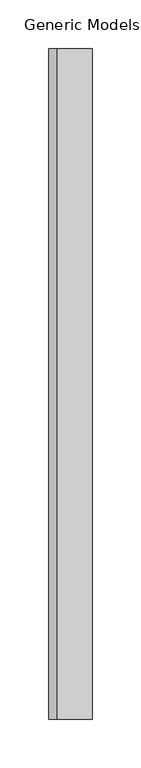
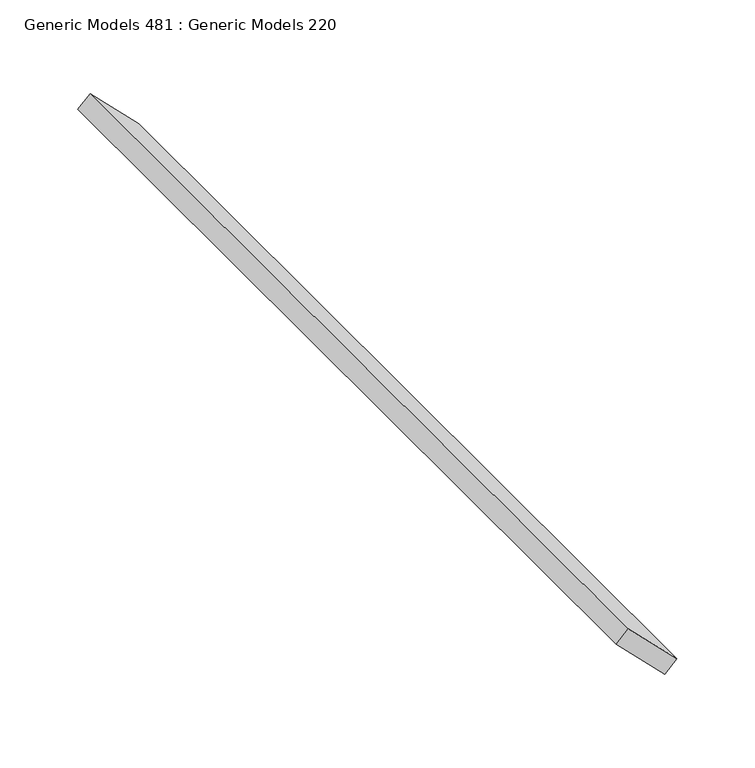
"""IFC4 building model written with IfcOpenShell, lengths in millimetres: proxy geometry, Generic Models 481 : Generic Models 220."""

from ifc_helpers import new_model, si_unit, frame, origin, place, context, project, spatial, polyline, outline, extrude, source, transform, mapped, element, save


def generic_models_481_generic_models_220_9f401b99(model_context):
    return source(origin(), model_context, "Body", "SweptSolid", [
        extrude(outline(polyline([(0.0, -50.8), (0.0, 0.0), (690.8142348, 0.0), (690.8142348, -50.8), (0.0, -50.8)])), frame((-6899.085451, -4564.8872686, 127815.1762561), z_axis=(0.7071067811865582, 0.0, 0.7071067811865369), x_axis=(0.0, 1.0, 0.0)), (0.0, 0.0, 1.0), 12.7),
    ])


if __name__ == "__main__":
    model = new_model("IFC4")
    model_context = context("Model", 3, world=origin())
    ifc_project = project(units=[si_unit("LENGTHUNIT", "METRE", prefix="MILLI")], contexts=[model_context])
    site = spatial("IfcSite", under=ifc_project)
    building = spatial("IfcBuilding", under=site)
    placement = place(None, origin())
    generic_models_481_generic_models_220_shape = generic_models_481_generic_models_220_9f401b99(model_context)
    element("IfcBuildingElementProxy", 1, Name="Generic Models 481 : Generic Models 220", ObjectType="Generic Models 481 : Generic Models 220", at=placement, inside=building, context=model_context, shape_type="MappedRepresentation", body=[
        mapped(generic_models_481_generic_models_220_shape, transform((0.0, 0.0, 0.0), x_axis=(1.0, 0.0, 0.0), y_axis=(0.0, 1.0, 0.0), z_axis=(0.0, 0.0, 1.0))),
    ])
    save(model, "model.ifc")

# Revit data of these elements
# Element 1 (IfcBuildingElementProxy, "Generic Models 481 : Generic Models 220")
#   Materials on its faces: "_WOOD TONE ALUMINUM EXTRUSION SLAT BY KNOTWOOD"
# Materials
#   "_WOOD TONE ALUMINUM EXTRUSION SLAT BY KNOTWOOD": class "Generic", colour RGB 177 130 114, transparency 0, Cost = 0
